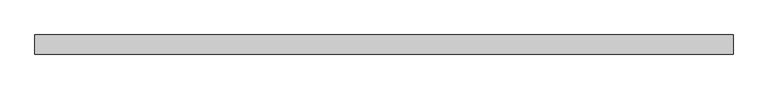
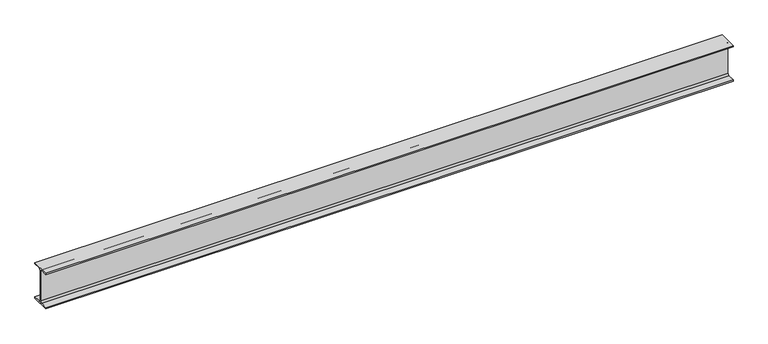
"""IFC4 building model written with IfcOpenShell, lengths in millimetres: beam geometry, 0912_Steel Framing_H-KSD3502 : H_SB_ASB_H-250x125x6x9."""

from ifc_helpers import new_model, si_unit, point, frame, frame_2d, origin, place, context, project, spatial, polyline, circle_curve, trimmed, segment, composite_curve, outline, extrude, source, transform, mapped, element, save


def beam_6b0b6d87(model_context):
    return source(origin(), model_context, "Body", "SweptSolid", [
        extrude(outline(composite_curve([segment(polyline([(62.5, -116.0), (62.5, -125.0), (-62.5, -125.0), (-62.5, -116.0), (-15.0, -116.0)]), True, "CONTINUOUS"), segment(trimmed(circle_curve(frame_2d((-15.0, -104.0)), 12.0), [point((-15.0, -116.0))], [point((-3.0, -104.0))], True, "CARTESIAN"), True, "CONTINUOUS"), segment(polyline([(-3.0, -104.0), (-3.0, 104.0)]), True, "CONTINUOUS"), segment(trimmed(circle_curve(frame_2d((-15.0, 104.0)), 12.0), [point((-3.0, 104.0))], [point((-15.0, 116.0))], True, "CARTESIAN"), True, "CONTINUOUS"), segment(polyline([(-15.0, 116.0), (-62.5, 116.0), (-62.5, 125.0), (62.5, 125.0), (62.5, 116.0), (15.0, 116.0)]), True, "CONTINUOUS"), segment(trimmed(circle_curve(frame_2d((15.0, 104.0)), 12.0), [point((15.0, 116.0))], [point((3.0, 104.0))], True, "CARTESIAN"), True, "CONTINUOUS"), segment(polyline([(3.0, 104.0), (3.0, -104.0)]), True, "CONTINUOUS"), segment(trimmed(circle_curve(frame_2d((15.0, -104.0)), 12.0), [point((3.0, -104.0))], [point((15.0, -116.0))], True, "CARTESIAN"), True, "CONTINUOUS"), segment(polyline([(15.0, -116.0), (62.5, -116.0)]), True, "CONTINUOUS")], self_intersect=False)), frame((-2404.8, 0.0, 0.0), z_axis=(1.0, 0.0, 0.0), x_axis=(0.0, 1.0, 0.0)), (0.0, 0.0, 1.0), 4569.2729123),
    ])


if __name__ == "__main__":
    model = new_model("IFC4")
    model_context = context("Model", 3, world=origin())
    ifc_project = project(units=[si_unit("LENGTHUNIT", "METRE", prefix="MILLI")], contexts=[model_context])
    site = spatial("IfcSite", under=ifc_project)
    building = spatial("IfcBuilding", under=site)
    placement = place(None, origin())
    beam_shape = beam_6b0b6d87(model_context)
    element("IfcBeam", 1, ObjectType="0912_Steel Framing_H-KSD3502 : H_SB_ASB_H-250x125x6x9", at=placement, inside=building, context=model_context, shape_type="MappedRepresentation", body=[
        mapped(beam_shape, transform((0.0, 0.0, 0.0), x_axis=(1.0, 0.0, 0.0), y_axis=(0.0, 1.0, 0.0), z_axis=(0.0, 0.0, 1.0))),
    ])
    save(model, "model.ifc")

# Revit data of these elements
# Type "0912_Steel Framing_H-KSD3502 : H_SB_ASB_H-250x125x6x9"
#   H_WM Code_1 = "S01AA003-00001 | Main Steel Structure Fabrication Work | Shelter/Building | Light Steel - Standard (30KG/M>Weight) | Material: (   )"
#   H_WM Code_2 = "S03AA029-00001 | Main Steel Structure Erection Work | Shelter/Building | Light Steel (30KG/M>Weight) | Material: (   )"
#   H_WM Code_3 = "S01AA010-00001 | Main Steel Structure Fabrication Work | Shelter/Building | Steel Painting/Coating | for Non-Fireproofed Steel Surface, Surface Preparation, Primer, Second & Final Coat | Material: (   )"
#   H_Q'ty Cal Type Tag = "SB-Q2"
#   Width = 12.5 cm
#   Web Thickness = 0.6 cm
#   Web Fillet = 1.2 cm
#   Warping Constant = 42539.8 cm⁶
#   W = 0
#   Torsional Moment of Inertia = 7.8102 cm⁴
#   Section Area = 37.66 cm²
#   Plastic Modulus weak axis = 73.1 cm³
#   Plastic Modulus strong axis = 366.0 cm³
#   Perimeter = 0.97 m²/m
#   Nominal Weight = 29.60 kgf/m
#   Moment of Inertia weak axis = 294.00 cm⁴
#   Moment of Inertia strong axis = 4050.00 cm⁴
#   Height = 25.0 cm
#   Flange Thickness = 0.9 cm
#   Elastic Modulus weak axis = 47.0 cm³
#   Elastic Modulus strong axis = 324.0 cm³
#   Centroid Vertical = 12.5 cm
#   Centroid Horizontal = 6.25 cm
#   Ix = 40500000
#   Length [instance default] = 1.5240 m
#   Zx = 366000
#   b = 0.1250 m
#   h = 0.2500 m
#   r = 0.0120 m
#   s = 0.0060 m
#   t = 0.0090 m
#   A = 0.003766 m²
#   Structural Material [instance default] = Steel, 45-345
#   Assembly Code = ""
# Element 1 (IfcBeam, "0912_Steel Framing_H-KSD3502 : H_SB_ASB_H-250x125x6x9")
#   Structural Material = none
# Materials
#   "Steel, 45-345": class "Metal", colour RGB 189 187 185, transparency 0, Description = "Steel 345 MPa", Cost = 0
